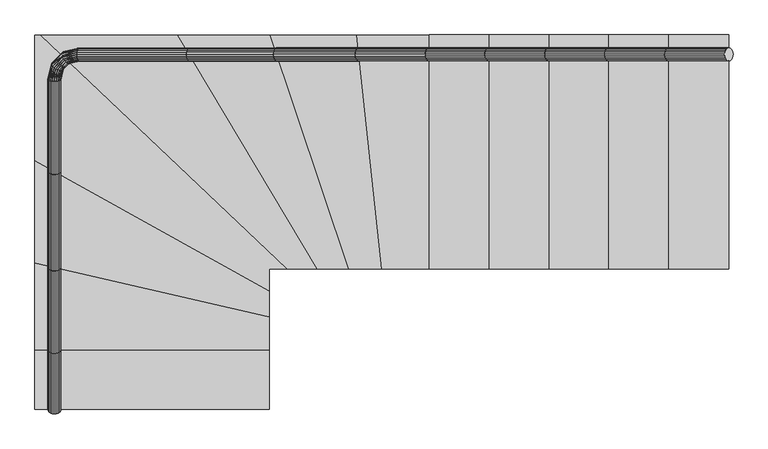
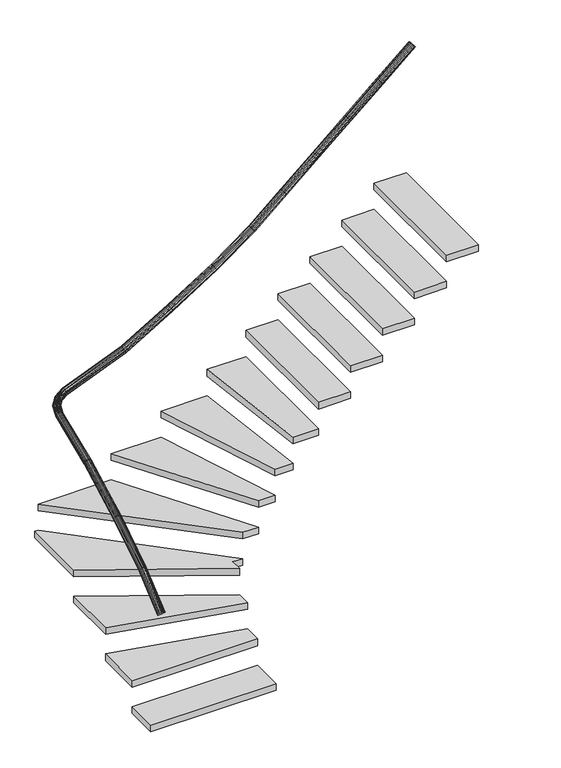
"""IFC4 building model written with IfcOpenShell, lengths in millimetres: stair geometry, 0_3d_modell."""

from ifc_helpers import new_model, si_unit, frame, origin, origin_with_axes, place, context, project, spatial, polyline, outline, extrude, faceted_brep, source, transform, mapped, element, save


def stair_df875d3e(model_context):
    return source(origin(), model_context, "Body", "SolidModel", [
        extrude(outline(polyline([(0.0, 246.9018591), (0.0, 579.8690495), (900.0, 373.9346688), (900.0, 246.9018591), (0.0, 246.9018591)])), frame((0.0, 0.0, 198.5714286), z_axis=(0.0, 0.0, 1.0), x_axis=(1.0, 0.0, 0.0)), (0.0, 0.0, 1.0), 50.0),
        extrude(outline(polyline([(0.0, 973.1970565), (0.0, 1456.9018591), (22.6704161, 1456.9018591), (970.0, 556.9018591), (900.0, 556.9018591), (900.0, 473.824936), (0.0, 973.1970565)])), frame((0.0, 0.0, 595.7142857), z_axis=(0.0, 0.0, 1.0), x_axis=(1.0, 0.0, 0.0)), (0.0, 0.0, 1.0), 50.0),
        extrude(outline(polyline([(548.8803485, 1456.9018591), (904.7220467, 1456.9018591), (1204.4816265, 556.9018591), (1084.3313864, 556.9018591), (548.8803485, 1456.9018591)])), frame((0.0, 0.0, 992.8571429), z_axis=(0.0, 0.0, 1.0), x_axis=(1.0, 0.0, 0.0)), (0.0, 0.0, 1.0), 50.0),
        faceted_brep([(98.7764129, 251.6675536, 1061.6862641), (100.0, 246.9018591, 1068.1306652), (98.7764129, 242.1361647, 1074.5750662), (95.2254249, 237.8369696, 1080.3886444), (89.6946313, 234.4251091, 1085.0023262), (82.7254249, 232.2345598, 1087.9644922), (75.0, 231.4797479, 1088.985185), (67.2745751, 232.2345598, 1087.9644922), (60.3053687, 234.4251091, 1085.0023262), (54.7745751, 237.8369696, 1080.3886444), (51.2235871, 242.1361647, 1074.5750662), (50.0, 246.9018591, 1068.1306652), (51.2235871, 251.6675536, 1061.6862641), (54.7745751, 255.9667486, 1055.872686), (60.3053687, 259.3786091, 1051.2590042), (67.2745751, 261.5691584, 1048.2968382), (75.0, 262.3239703, 1047.2761453), (82.7254249, 261.5691584, 1048.2968382), (89.6946313, 259.3786091, 1051.2590042), (95.2254249, 255.9667486, 1055.872686), (98.7764129, 558.6819455, 1273.6116568), (100.0, 562.7078511, 1266.7020937), (98.7764129, 566.7337566, 1259.7925307), (95.2254249, 570.3655785, 1253.5593239), (89.6946313, 573.2478087, 1248.6126229), (82.7254249, 575.0983143, 1245.4366454), (75.0, 575.7359551, 1244.3422781), (67.2745751, 575.0983143, 1245.4366454), (60.3053687, 573.2478087, 1248.6126229), (54.7745751, 570.3655785, 1253.5593239), (51.2235871, 566.7337566, 1259.7925307), (50.0, 562.7078511, 1266.7020937), (51.2235871, 558.6819455, 1273.6116568), (54.7745751, 555.0501237, 1279.8448636), (60.3053687, 552.1678935, 1284.7915646), (67.2745751, 550.3173878, 1287.9675421), (75.0, 549.679747, 1289.0619094), (82.7254249, 550.3173878, 1287.9675421), (89.6946313, 552.1678935, 1284.7915646), (95.2254249, 555.0501237, 1279.8448636)], [[[0, 1, 2, 3, 4, 5, 6, 7, 8, 9, 10, 11, 12, 13, 14, 15, 16, 17, 18, 19]], [[20, 21, 22, 23, 24, 25, 26, 27, 28, 29, 30, 31, 32, 33, 34, 35, 36, 37, 38, 39]], [[2, 1, 21, 20]], [[3, 2, 20, 39]], [[4, 3, 39, 38]], [[5, 4, 38, 37]], [[6, 5, 37, 36]], [[7, 6, 36, 35]], [[8, 7, 35, 34]], [[9, 8, 34, 33]], [[10, 9, 33, 32]], [[11, 10, 32, 31]], [[12, 11, 31, 30]], [[13, 12, 30, 29]], [[14, 13, 29, 28]], [[15, 14, 28, 27]], [[16, 15, 27, 26]], [[17, 16, 26, 25]], [[18, 17, 25, 24]], [[19, 18, 24, 23]], [[0, 19, 23, 22]], [[1, 0, 22, 21]]]),
        extrude(outline(polyline([(1974.6018366, 1456.9018591), (2204.6018366, 1456.9018591), (2204.6018366, 556.9018591), (1974.6018366, 556.9018591), (1974.6018366, 1456.9018591)])), frame((0.0, 0.0, 1985.7142857), z_axis=(0.0, 0.0, 1.0), x_axis=(1.0, 0.0, 0.0)), (0.0, 0.0, 1.0), 50.0),
        extrude(outline(polyline([(1.2235871, -7.9923214), (0.0, 0.0), (1.2235871, 7.9923214), (4.7745752, 15.2022986), (10.3053687, 20.9241691), (17.2745752, 24.5978359), (25.0, 25.8636953), (32.7254249, 24.5978359), (39.6946313, 20.9241691), (45.2254249, 15.2022986), (48.7764129, 7.9923214), (50.0, 0.0), (48.7764129, -7.9923214), (45.2254249, -15.2022986), (39.6946313, -20.9241691), (32.7254249, -24.5978359), (25.0, -25.8636953), (17.2745752, -24.5978359), (10.3053687, -20.9241691), (4.7745752, -15.2022986), (1.2235871, -7.9923214)])), frame((2204.6018366, 1356.9018591, 3053.8449509), z_axis=(0.7569287102857765, 0.0, 0.6534974579484691), x_axis=(0.0, 1.0, 0.0)), (0.0, 0.0, 1.0), 303.8595272),
        faceted_brep([(98.7764129, 566.7337566, 1259.7925307), (100.0, 562.7078511, 1266.7020937), (98.7764129, 558.6819455, 1273.6116568), (95.2254249, 555.0501237, 1279.8448636), (89.6946313, 552.1678935, 1284.7915646), (82.7254249, 550.3173878, 1287.9675421), (75.0, 549.679747, 1289.0619094), (67.2745751, 550.3173878, 1287.9675421), (60.3053687, 552.1678935, 1284.7915646), (54.7745751, 555.0501237, 1279.8448636), (51.2235871, 558.6819455, 1273.6116568), (50.0, 562.7078511, 1266.7020937), (51.2235871, 566.7337566, 1259.7925307), (54.7745751, 570.3655785, 1253.5593239), (60.3053687, 573.2478087, 1248.6126229), (67.2745751, 575.0983143, 1245.4366454), (75.0, 575.7359551, 1244.3422781), (82.7254249, 575.0983143, 1245.4366454), (89.6946313, 573.2478087, 1248.6126229), (95.2254249, 570.3655785, 1253.5593239), (98.7764129, 928.1440687, 1472.4992177), (100.0, 931.5827131, 1465.2735223), (98.7764129, 935.0213576, 1458.0478269), (95.2254249, 938.1234035, 1451.529433), (89.6946313, 940.5852011, 1446.3564062), (82.7254249, 942.1657724, 1443.0351186), (75.0, 942.7104002, 1441.8906809), (67.2745751, 942.1657724, 1443.0351186), (60.3053687, 940.5852011, 1446.3564062), (54.7745751, 938.1234035, 1451.529433), (51.2235871, 935.0213576, 1458.0478269), (50.0, 931.5827131, 1465.2735223), (51.2235871, 928.1440687, 1472.4992177), (54.7745751, 925.0420228, 1479.0176117), (60.3053687, 922.5802252, 1484.1906384), (67.2745751, 920.9996538, 1487.511926), (75.0, 920.4550261, 1488.6563638), (82.7254249, 920.9996538, 1487.511926), (89.6946313, 922.5802252, 1484.1906384), (95.2254249, 925.0420228, 1479.0176117)], [[[0, 1, 2, 3, 4, 5, 6, 7, 8, 9, 10, 11, 12, 13, 14, 15, 16, 17, 18, 19]], [[20, 21, 22, 23, 24, 25, 26, 27, 28, 29, 30, 31, 32, 33, 34, 35, 36, 37, 38, 39]], [[2, 1, 21, 20]], [[3, 2, 20, 39]], [[4, 3, 39, 38]], [[5, 4, 38, 37]], [[6, 5, 37, 36]], [[7, 6, 36, 35]], [[8, 7, 35, 34]], [[9, 8, 34, 33]], [[10, 9, 33, 32]], [[11, 10, 32, 31]], [[12, 11, 31, 30]], [[13, 12, 30, 29]], [[14, 13, 29, 28]], [[15, 14, 28, 27]], [[16, 15, 27, 26]], [[17, 16, 26, 25]], [[18, 17, 25, 24]], [[19, 18, 24, 23]], [[0, 19, 23, 22]], [[1, 0, 22, 21]]]),
        extrude(outline(polyline([(2434.6018366, 1456.9018591), (2664.6018366, 1456.9018591), (2664.6018366, 556.9018591), (2434.6018366, 556.9018591), (2434.6018366, 1456.9018591)])), frame((0.0, 0.0, 2382.8571429), z_axis=(0.0, 0.0, 1.0), x_axis=(1.0, 0.0, 0.0)), (0.0, 0.0, 1.0), 50.0),
        faceted_brep([(98.7764129, 935.0213576, 1458.0478269), (100.0, 931.5827131, 1465.2735223), (98.7764129, 928.1440687, 1472.4992177), (95.2254249, 925.0420228, 1479.0176117), (89.6946313, 922.5802252, 1484.1906384), (82.7254249, 920.9996538, 1487.511926), (75.0, 920.4550261, 1488.6563638), (67.2745751, 920.9996538, 1487.511926), (60.3053687, 922.5802252, 1484.1906384), (54.7745751, 925.0420228, 1479.0176117), (51.2235871, 928.1440687, 1472.4992177), (50.0, 931.5827131, 1465.2735223), (51.2235871, 935.0213576, 1458.0478269), (54.7745751, 938.1234035, 1451.529433), (60.3053687, 940.5852011, 1446.3564062), (67.2745751, 942.1657724, 1443.0351186), (75.0, 942.7104002, 1441.8906809), (82.7254249, 942.1657724, 1443.0351186), (89.6946313, 940.5852011, 1446.3564062), (95.2254249, 938.1234035, 1451.529433), (98.7764129, 1283.3224302, 1620.3777918), (100.0, 1286.3944101, 1612.9994356), (98.7764129, 1289.46639, 1605.6210794), (95.2254249, 1292.2376632, 1598.9649681), (89.6946313, 1294.436958, 1593.6826483), (82.7254249, 1295.8489921, 1590.2911902), (75.0, 1296.335546, 1589.1225734), (67.2745751, 1295.8489921, 1590.2911902), (60.3053687, 1294.436958, 1593.6826483), (54.7745751, 1292.2376632, 1598.9649681), (51.2235871, 1289.46639, 1605.6210794), (50.0, 1286.3944101, 1612.9994356), (51.2235871, 1283.3224302, 1620.3777918), (54.7745751, 1280.5511571, 1627.0339031), (60.3053687, 1278.3518623, 1632.3162229), (67.2745751, 1276.9398281, 1635.707681), (75.0, 1276.4532743, 1636.8762979), (82.7254249, 1276.9398281, 1635.707681), (89.6946313, 1278.3518623, 1632.3162229), (95.2254249, 1280.5511571, 1627.0339031)], [[[0, 1, 2, 3, 4, 5, 6, 7, 8, 9, 10, 11, 12, 13, 14, 15, 16, 17, 18, 19]], [[20, 21, 22, 23, 24, 25, 26, 27, 28, 29, 30, 31, 32, 33, 34, 35, 36, 37, 38, 39]], [[2, 1, 21, 20]], [[3, 2, 20, 39]], [[4, 3, 39, 38]], [[5, 4, 38, 37]], [[6, 5, 37, 36]], [[7, 6, 36, 35]], [[8, 7, 35, 34]], [[9, 8, 34, 33]], [[10, 9, 33, 32]], [[11, 10, 32, 31]], [[12, 11, 31, 30]], [[13, 12, 30, 29]], [[14, 13, 29, 28]], [[15, 14, 28, 27]], [[16, 15, 27, 26]], [[17, 16, 26, 25]], [[18, 17, 25, 24]], [[19, 18, 24, 23]], [[0, 19, 23, 22]], [[1, 0, 22, 21]]]),
        faceted_brep([(1249.3489942, 1358.1254462, 2252.9513864), (1244.8437697, 1356.9018591, 2259.5592366), (1240.3385453, 1358.1254462, 2266.1670868), (1236.2743236, 1361.6764343, 2272.1281145), (1233.048939, 1367.2072278, 2276.858813), (1230.9781146, 1374.1764343, 2279.8961083), (1230.2645572, 1381.9018591, 2280.942689), (1230.9781146, 1389.627284, 2279.8961083), (1233.048939, 1396.5964904, 2276.858813), (1236.2743236, 1402.127284, 2272.1281145), (1240.3385453, 1405.678272, 2266.1670868), (1244.8437697, 1406.9018591, 2259.5592366), (1249.3489942, 1405.678272, 2252.9513864), (1253.4132159, 1402.127284, 2246.9903587), (1256.6386004, 1396.5964904, 2242.2596602), (1258.7094248, 1389.627284, 2239.2223649), (1259.4229823, 1381.9018591, 2238.1757842), (1258.7094248, 1374.1764343, 2239.2223649), (1256.6386004, 1367.2072278, 2242.2596602), (1253.4132159, 1361.6764343, 2246.9903587), (1509.6138519, 1358.1254462, 2464.383151), (1514.6018366, 1356.9018591, 2458.1306652), (1519.5898213, 1358.1254462, 2451.8781793), (1524.0895473, 1361.6764343, 2446.2377304), (1527.6605501, 1367.2072278, 2441.7614447), (1529.9532751, 1374.1764343, 2438.8874925), (1530.7432942, 1381.9018591, 2437.897196), (1529.9532751, 1389.627284, 2438.8874925), (1527.6605501, 1396.5964904, 2441.7614447), (1524.0895473, 1402.127284, 2446.2377304), (1519.5898213, 1405.678272, 2451.8781793), (1514.6018366, 1406.9018591, 2458.1306652), (1509.6138519, 1405.678272, 2464.383151), (1505.1141259, 1402.127284, 2470.0236), (1501.5431231, 1396.5964904, 2474.4998856), (1499.2503981, 1389.627284, 2477.3738379), (1498.460379, 1381.9018591, 2478.3641344), (1499.2503981, 1374.1764343, 2477.3738379), (1501.5431231, 1367.2072278, 2474.4998856), (1505.1141259, 1361.6764343, 2470.0236)], [[[0, 1, 2, 3, 4, 5, 6, 7, 8, 9, 10, 11, 12, 13, 14, 15, 16, 17, 18, 19]], [[20, 21, 22, 23, 24, 25, 26, 27, 28, 29, 30, 31, 32, 33, 34, 35, 36, 37, 38, 39]], [[2, 1, 21, 20]], [[3, 2, 20, 39]], [[4, 3, 39, 38]], [[5, 4, 38, 37]], [[6, 5, 37, 36]], [[7, 6, 36, 35]], [[8, 7, 35, 34]], [[9, 8, 34, 33]], [[10, 9, 33, 32]], [[11, 10, 32, 31]], [[12, 11, 31, 30]], [[13, 12, 30, 29]], [[14, 13, 29, 28]], [[15, 14, 28, 27]], [[16, 15, 27, 26]], [[17, 16, 26, 25]], [[18, 17, 25, 24]], [[19, 18, 24, 23]], [[0, 19, 23, 22]], [[1, 0, 22, 21]]]),
        extrude(outline(polyline([(1.2235871, -7.9923214), (0.0, 0.0), (1.2235871, 7.9923214), (4.7745752, 15.2022986), (10.3053687, 20.924169), (17.2745752, 24.5978359), (25.0, 25.8636953), (32.7254249, 24.5978359), (39.6946313, 20.924169), (45.2254249, 15.2022986), (48.7764129, 7.9923214), (50.0, 0.0), (48.7764129, -7.9923214), (45.2254249, -15.2022986), (39.6946313, -20.9241691), (32.7254249, -24.597836), (25.0, -25.8636953), (17.2745752, -24.597836), (10.3053687, -20.9241691), (4.7745752, -15.2022986), (1.2235871, -7.9923214)])), frame((2434.6018366, 1356.9018591, 3252.4163795), z_axis=(0.7569287102857786, 0.0, 0.6534974579484667), x_axis=(0.0, 1.0, 0.0)), (0.0, 0.0, 1.0), 303.8595272),
        extrude(outline(polyline([(0.0, 579.8690495), (0.0, 973.1970565), (900.0, 473.824936), (900.0, 373.9346688), (0.0, 579.8690495)])), frame((0.0, 0.0, 397.1428571), z_axis=(0.0, 0.0, 1.0), x_axis=(1.0, 0.0, 0.0)), (0.0, 0.0, 1.0), 50.0),
        extrude(outline(polyline([(22.6704161, 1456.9018591), (548.8803485, 1456.9018591), (1084.3313864, 556.9018591), (970.0, 556.9018591), (22.6704161, 1456.9018591)])), frame((0.0, 0.0, 794.2857143), z_axis=(0.0, 0.0, 1.0), x_axis=(1.0, 0.0, 0.0)), (0.0, 0.0, 1.0), 50.0),
        extrude(outline(polyline([(1.2235871, -7.9923214), (0.0, 0.0), (1.2235871, 7.9923214), (4.7745752, 15.2022987), (10.3053687, 20.9241691), (17.2745752, 24.597836), (25.0, 25.8636953), (32.7254249, 24.597836), (39.6946313, 20.9241691), (45.2254249, 15.2022987), (48.7764129, 7.9923214), (50.0, 0.0), (48.7764129, -7.9923214), (45.2254249, -15.2022986), (39.6946313, -20.924169), (32.7254249, -24.5978359), (25.0, -25.8636953), (17.2745752, -24.5978359), (10.3053687, -20.924169), (4.7745752, -15.2022986), (1.2235871, -7.9923214)])), frame((1744.6018366, 1356.9018591, 2656.7020937), z_axis=(0.7569287102857375, 0.0, 0.6534974579485143), x_axis=(0.0, 1.0, 0.0)), (0.0, 0.0, 1.0), 303.8595272),
        faceted_brep([(933.8654844, 1358.1254462, 2054.1646194), (929.7020117, 1356.9018591, 2060.987808), (925.538539, 1358.1254462, 2067.8109967), (921.782616, 1361.6764343, 2073.966284), (918.8018987, 1367.2072278, 2078.8511477), (916.8881603, 1374.1764343, 2081.9874233), (916.228731, 1381.9018591, 2083.0681102), (916.8881603, 1389.627284, 2081.9874233), (918.8018987, 1396.5964904, 2078.8511477), (921.782616, 1402.127284, 2073.966284), (925.538539, 1405.678272, 2067.8109967), (929.7020117, 1406.9018591, 2060.987808), (933.8654844, 1405.678272, 2054.1646194), (937.6214074, 1402.127284, 2048.009332), (940.6021247, 1396.5964904, 2043.1244683), (942.515863, 1389.627284, 2039.9881928), (943.1752923, 1381.9018591, 2038.9075058), (942.515863, 1374.1764343, 2039.9881928), (940.6021247, 1367.2072278, 2043.1244683), (937.6214074, 1361.6764343, 2048.009332), (1240.3385453, 1358.1254462, 2266.1670868), (1244.8437697, 1356.9018591, 2259.5592366), (1249.3489942, 1358.1254462, 2252.9513864), (1253.4132159, 1361.6764343, 2246.9903587), (1256.6386004, 1367.2072278, 2242.2596602), (1258.7094248, 1374.1764343, 2239.2223649), (1259.4229823, 1381.9018591, 2238.1757842), (1258.7094248, 1389.627284, 2239.2223649), (1256.6386004, 1396.5964904, 2242.2596602), (1253.4132159, 1402.127284, 2246.9903587), (1249.3489942, 1405.678272, 2252.9513864), (1244.8437697, 1406.9018591, 2259.5592366), (1240.3385453, 1405.678272, 2266.1670868), (1236.2743236, 1402.127284, 2272.1281145), (1233.048939, 1396.5964904, 2276.858813), (1230.9781146, 1389.627284, 2279.8961083), (1230.2645572, 1381.9018591, 2280.942689), (1230.9781146, 1374.1764343, 2279.8961083), (1233.048939, 1367.2072278, 2276.858813), (1236.2743236, 1361.6764343, 2272.1281145)], [[[0, 1, 2, 3, 4, 5, 6, 7, 8, 9, 10, 11, 12, 13, 14, 15, 16, 17, 18, 19]], [[20, 21, 22, 23, 24, 25, 26, 27, 28, 29, 30, 31, 32, 33, 34, 35, 36, 37, 38, 39]], [[2, 1, 21, 20]], [[3, 2, 20, 39]], [[4, 3, 39, 38]], [[5, 4, 38, 37]], [[6, 5, 37, 36]], [[7, 6, 36, 35]], [[8, 7, 35, 34]], [[9, 8, 34, 33]], [[10, 9, 33, 32]], [[11, 10, 32, 31]], [[12, 11, 31, 30]], [[13, 12, 30, 29]], [[14, 13, 29, 28]], [[15, 14, 28, 27]], [[16, 15, 27, 26]], [[17, 16, 26, 25]], [[18, 17, 25, 24]], [[19, 18, 24, 23]], [[0, 19, 23, 22]], [[1, 0, 22, 21]]]),
        faceted_brep([(597.0493296, 1358.1254462, 1855.2297082), (593.5012683, 1356.9018591, 1862.4163795), (589.9532071, 1358.1254462, 1869.6030507), (586.7524548, 1361.6764343, 1876.0862405), (584.2123234, 1367.2072278, 1881.231329), (582.5814586, 1374.1764343, 1884.5346792), (582.019501, 1381.9018591, 1885.6729361), (582.5814586, 1389.627284, 1884.5346792), (584.2123234, 1396.5964904, 1881.231329), (586.7524548, 1402.127284, 1876.0862405), (589.9532071, 1405.678272, 1869.6030507), (593.5012683, 1406.9018591, 1862.4163795), (597.0493296, 1405.678272, 1855.2297082), (600.2500819, 1402.127284, 1848.7465184), (602.7902133, 1396.5964904, 1843.6014299), (604.421078, 1389.627284, 1840.2980797), (604.9830357, 1381.9018591, 1839.1598228), (604.421078, 1374.1764343, 1840.2980797), (602.7902133, 1367.2072278, 1843.6014299), (600.2500819, 1361.6764343, 1848.7465184), (925.538539, 1358.1254462, 2067.8109967), (929.7020117, 1356.9018591, 2060.987808), (933.8654844, 1358.1254462, 2054.1646194), (937.6214074, 1361.6764343, 2048.009332), (940.6021247, 1367.2072278, 2043.1244683), (942.515863, 1374.1764343, 2039.9881928), (943.1752923, 1381.9018591, 2038.9075058), (942.515863, 1389.627284, 2039.9881928), (940.6021247, 1396.5964904, 2043.1244683), (937.6214074, 1402.127284, 2048.009332), (933.8654844, 1405.678272, 2054.1646194), (929.7020117, 1406.9018591, 2060.987808), (925.538539, 1405.678272, 2067.8109967), (921.782616, 1402.127284, 2073.966284), (918.8018987, 1396.5964904, 2078.8511477), (916.8881603, 1389.627284, 2081.9874233), (916.228731, 1381.9018591, 2083.0681102), (916.8881603, 1374.1764343, 2081.9874233), (918.8018987, 1367.2072278, 2078.8511477), (921.782616, 1361.6764343, 2073.966284)], [[[0, 1, 2, 3, 4, 5, 6, 7, 8, 9, 10, 11, 12, 13, 14, 15, 16, 17, 18, 19]], [[20, 21, 22, 23, 24, 25, 26, 27, 28, 29, 30, 31, 32, 33, 34, 35, 36, 37, 38, 39]], [[2, 1, 21, 20]], [[3, 2, 20, 39]], [[4, 3, 39, 38]], [[5, 4, 38, 37]], [[6, 5, 37, 36]], [[7, 6, 36, 35]], [[8, 7, 35, 34]], [[9, 8, 34, 33]], [[10, 9, 33, 32]], [[11, 10, 32, 31]], [[12, 11, 31, 30]], [[13, 12, 30, 29]], [[14, 13, 29, 28]], [[15, 14, 28, 27]], [[16, 15, 27, 26]], [[17, 16, 26, 25]], [[18, 17, 25, 24]], [[19, 18, 24, 23]], [[0, 19, 23, 22]], [[1, 0, 22, 21]]]),
        faceted_brep([(98.7764129, 1289.46639, 1605.6210794), (100.0, 1286.3944101, 1612.9994356), (98.7764129, 1283.3224302, 1620.3777918), (95.2254249, 1280.5511571, 1627.0339031), (89.6946313, 1278.3518623, 1632.3162229), (82.7254249, 1276.9398281, 1635.707681), (75.0, 1276.4532743, 1636.8762979), (67.2745751, 1276.9398281, 1635.707681), (60.3053687, 1278.3518623, 1632.3162229), (54.7745751, 1280.5511571, 1627.0339031), (51.2235871, 1283.3224302, 1620.3777918), (50.0, 1286.3944101, 1612.9994356), (51.2235871, 1289.46639, 1605.6210794), (54.7745751, 1292.2376632, 1598.9649681), (60.3053687, 1294.436958, 1593.6826483), (67.2745751, 1295.8489921, 1590.2911902), (75.0, 1296.335546, 1589.1225734), (82.7254249, 1295.8489921, 1590.2911902), (89.6946313, 1294.436958, 1593.6826483), (95.2254249, 1292.2376632, 1598.9649681), (108.8679012, 1324.8479302, 1638.9123688), (105.9144976, 1321.9997167, 1645.879395), (101.1034244, 1320.6050585, 1652.1644401), (94.9056231, 1320.8004745, 1657.1522801), (87.9277774, 1322.5668359, 1660.3546705), (80.8529277, 1325.7312391, 1661.4581391), (74.3736094, 1329.9839302, 1660.3546705), (69.1240635, 1334.9086261, 1657.1522801), (65.6181519, 1340.0232633, 1652.1644401), (64.1990579, 1344.8271855, 1645.879395), (65.0056921, 1348.8501513, 1638.9123688), (67.9590957, 1351.6983647, 1631.9453426), (72.7701688, 1353.0930229, 1625.6602975), (78.9679702, 1352.8976069, 1620.6724574), (85.9458159, 1351.1312455, 1617.470067), (93.0206656, 1347.9668423, 1616.3665985), (99.4999839, 1343.7141513, 1617.470067), (104.7495298, 1338.7894554, 1620.6724574), (108.2554414, 1333.6748181, 1625.6602975), (109.6745354, 1328.870896, 1631.9453426), (132.1170605, 1348.0291684, 1666.2859781), (128.1175831, 1347.2454175, 1673.2691208), (123.3397137, 1348.6878091, 1679.5687049), (118.2511434, 1352.215152, 1684.5680831), (113.3499769, 1357.4821652, 1687.7778814), (109.1159746, 1363.9732768, 1688.8839026), (105.96359, 1371.0530916, 1687.7778814), (104.2014005, 1378.028588, 1684.5680831), (104.0019016, 1384.2169558, 1679.5687049), (105.3846216, 1389.0124344, 1673.2691208), (108.2142101, 1391.9456089, 1666.2859781), (112.2136875, 1392.7293599, 1659.3028354), (116.9915569, 1391.2869683, 1653.0032514), (122.0801271, 1387.7596254, 1648.0038732), (126.9812936, 1382.4926122, 1644.7940748), (131.215296, 1376.0015006, 1643.6880537), (134.3676806, 1368.9216857, 1644.7940748), (136.1298701, 1361.9461894, 1648.0038732), (136.329369, 1355.7578216, 1653.0032514), (134.946649, 1350.962343, 1659.3028354), (170.8141891, 1356.9018591, 1691.7803901), (167.8223333, 1358.1254462, 1699.1915978), (165.1233413, 1361.6764343, 1705.8773449), (162.981409, 1367.2072278, 1711.1831838), (161.6062039, 1374.1764343, 1714.5897421), (161.1323405, 1381.9018591, 1715.7635621), (161.6062039, 1389.627284, 1714.5897421), (162.981409, 1396.5964904, 1711.1831838), (165.1233413, 1402.127284, 1705.8773449), (167.8223333, 1405.678272, 1699.1915978), (170.8141891, 1406.9018591, 1691.7803901), (173.8060448, 1405.678272, 1684.3691823), (176.5050369, 1402.127284, 1677.6834352), (178.6469691, 1396.5964904, 1672.3775963), (180.0221742, 1389.627284, 1668.971038), (180.4960376, 1381.9018591, 1667.797218), (180.0221742, 1374.1764343, 1668.971038), (178.6469691, 1367.2072278, 1672.3775963), (176.5050369, 1361.6764343, 1677.6834352), (173.8060448, 1358.1254462, 1684.3691823), (589.9532071, 1358.1254462, 1869.6030507), (593.5012683, 1356.9018591, 1862.4163795), (597.0493296, 1358.1254462, 1855.2297082), (600.2500819, 1361.6764343, 1848.7465184), (602.7902133, 1367.2072278, 1843.6014299), (604.421078, 1374.1764343, 1840.2980797), (604.9830357, 1381.9018591, 1839.1598228), (604.421078, 1389.627284, 1840.2980797), (602.7902133, 1396.5964904, 1843.6014299), (600.2500819, 1402.127284, 1848.7465184), (597.0493296, 1405.678272, 1855.2297082), (593.5012683, 1406.9018591, 1862.4163795), (589.9532071, 1405.678272, 1869.6030507), (586.7524548, 1402.127284, 1876.0862405), (584.2123234, 1396.5964904, 1881.231329), (582.5814586, 1389.627284, 1884.5346792), (582.019501, 1381.9018591, 1885.6729361), (582.5814586, 1374.1764343, 1884.5346792), (584.2123234, 1367.2072278, 1881.231329), (586.7524548, 1361.6764343, 1876.0862405)], [[[0, 1, 2, 3, 4, 5, 6, 7, 8, 9, 10, 11, 12, 13, 14, 15, 16, 17, 18, 19]], [[2, 1, 20]], [[21, 2, 20]], [[3, 2, 21]], [[22, 3, 21]], [[4, 3, 22]], [[23, 4, 22]], [[5, 4, 23]], [[24, 5, 23]], [[6, 5, 24]], [[25, 6, 24]], [[7, 6, 25]], [[26, 7, 25]], [[8, 7, 26]], [[27, 8, 26]], [[9, 8, 27]], [[28, 9, 27]], [[10, 9, 28]], [[29, 10, 28]], [[11, 10, 29]], [[30, 11, 29]], [[12, 11, 30]], [[31, 12, 30]], [[13, 12, 31]], [[32, 13, 31]], [[14, 13, 32]], [[33, 14, 32]], [[15, 14, 33]], [[34, 15, 33]], [[16, 15, 34]], [[35, 16, 34]], [[17, 16, 35]], [[36, 17, 35]], [[18, 17, 36]], [[37, 18, 36]], [[19, 18, 37]], [[38, 19, 37]], [[0, 19, 38]], [[39, 0, 38]], [[1, 0, 39]], [[20, 1, 39]], [[21, 20, 40]], [[41, 21, 40]], [[22, 21, 41]], [[42, 22, 41]], [[23, 22, 42]], [[43, 23, 42]], [[24, 23, 43]], [[44, 24, 43]], [[25, 24, 44]], [[45, 25, 44]], [[26, 25, 45]], [[46, 26, 45]], [[27, 26, 46]], [[47, 27, 46]], [[28, 27, 47]], [[48, 28, 47]], [[29, 28, 48]], [[49, 29, 48]], [[30, 29, 49]], [[50, 30, 49]], [[31, 30, 50]], [[51, 31, 50]], [[32, 31, 51]], [[52, 32, 51]], [[33, 32, 52]], [[53, 33, 52]], [[34, 33, 53]], [[54, 34, 53]], [[35, 34, 54]], [[55, 35, 54]], [[36, 35, 55]], [[56, 36, 55]], [[37, 36, 56]], [[57, 37, 56]], [[38, 37, 57]], [[58, 38, 57]], [[39, 38, 58]], [[59, 39, 58]], [[20, 39, 59]], [[40, 20, 59]], [[41, 40, 60]], [[61, 41, 60]], [[42, 41, 61]], [[62, 42, 61]], [[43, 42, 62]], [[63, 43, 62]], [[44, 43, 63]], [[64, 44, 63]], [[45, 44, 64]], [[65, 45, 64]], [[46, 45, 65]], [[66, 46, 65]], [[47, 46, 66]], [[67, 47, 66]], [[48, 47, 67]], [[68, 48, 67]], [[49, 48, 68]], [[69, 49, 68]], [[50, 49, 69]], [[70, 50, 69]], [[51, 50, 70]], [[71, 51, 70]], [[52, 51, 71]], [[72, 52, 71]], [[53, 52, 72]], [[73, 53, 72]], [[54, 53, 73]], [[74, 54, 73]], [[55, 54, 74]], [[75, 55, 74]], [[56, 55, 75]], [[76, 56, 75]], [[57, 56, 76]], [[77, 57, 76]], [[58, 57, 77]], [[78, 58, 77]], [[59, 58, 78]], [[79, 59, 78]], [[40, 59, 79]], [[60, 40, 79]], [[80, 81, 82, 83, 84, 85, 86, 87, 88, 89, 90, 91, 92, 93, 94, 95, 96, 97, 98, 99]], [[61, 60, 81, 80]], [[62, 61, 80, 99]], [[63, 62, 99, 98]], [[64, 63, 98, 97]], [[65, 64, 97, 96]], [[66, 65, 96, 95]], [[67, 66, 95, 94]], [[68, 67, 94, 93]], [[69, 68, 93, 92]], [[70, 69, 92, 91]], [[71, 70, 91, 90]], [[72, 71, 90, 89]], [[73, 72, 89, 88]], [[74, 73, 88, 87]], [[75, 74, 87, 86]], [[76, 75, 86, 85]], [[77, 76, 85, 84]], [[78, 77, 84, 83]], [[79, 78, 83, 82]], [[60, 79, 82, 81]]]),
        extrude(outline(polyline([(1.2235871, -7.9923214), (0.0, 0.0), (1.2235871, 7.9923214), (4.7745752, 15.2022986), (10.3053687, 20.9241691), (17.2745752, 24.5978359), (25.0, 25.8636953), (32.7254249, 24.5978359), (39.6946313, 20.9241691), (45.2254249, 15.2022986), (48.7764129, 7.9923214), (50.0, 0.0), (48.7764129, -7.9923214), (45.2254249, -15.2022986), (39.6946313, -20.924169), (32.7254249, -24.5978359), (25.0, -25.8636953), (17.2745752, -24.5978359), (10.3053687, -20.924169), (4.7745752, -15.2022986), (1.2235871, -7.9923214)])), frame((1974.6018366, 1356.9018591, 2855.2735223), z_axis=(0.7569287102857345, 0.0, 0.6534974579485179), x_axis=(0.0, 1.0, 0.0)), (0.0, 0.0, 1.0), 303.8595272),
        extrude(outline(polyline([(0.0, 16.9018591), (0.0, 246.9018591), (900.0, 246.9018591), (900.0, 16.9018591), (0.0, 16.9018591)])), origin_with_axes(), (0.0, 0.0, 1.0), 50.0),
        extrude(outline(polyline([(1744.6018366, 1456.9018591), (1974.6018366, 1456.9018591), (1974.6018366, 556.9018591), (1744.6018366, 556.9018591), (1744.6018366, 1456.9018591)])), frame((0.0, 0.0, 1787.1428571), z_axis=(0.0, 0.0, 1.0), x_axis=(1.0, 0.0, 0.0)), (0.0, 0.0, 1.0), 50.0),
        faceted_brep([(98.7764129, 22.1248208, 863.5096191), (100.0, 16.9018591, 869.5592366), (98.7764129, 11.6788974, 875.6088541), (95.2254249, 6.9671956, 881.0662929), (89.6946313, 3.2279679, 885.3973409), (82.7254249, 0.8272359, 888.1780448), (75.0, 0.0, 889.1362101), (67.2745751, 0.8272359, 888.1780448), (60.3053687, 3.2279679, 885.3973409), (54.7745751, 6.9671956, 881.0662929), (51.2235871, 11.6788974, 875.6088541), (50.0, 16.9018591, 869.5592366), (51.2235871, 22.1248208, 863.5096191), (54.7745751, 26.8365226, 858.0521803), (60.3053687, 30.5757504, 853.7211323), (67.2745751, 32.9764824, 850.9404284), (75.0, 33.8037182, 849.9822631), (82.7254249, 32.9764824, 850.9404284), (89.6946313, 30.5757504, 853.7211323), (95.2254249, 26.8365226, 858.0521803), (98.7764129, 242.1361647, 1074.5750662), (100.0, 246.9018591, 1068.1306652), (98.7764129, 251.6675536, 1061.6862641), (95.2254249, 255.9667486, 1055.872686), (89.6946313, 259.3786091, 1051.2590042), (82.7254249, 261.5691584, 1048.2968382), (75.0, 262.3239703, 1047.2761453), (67.2745751, 261.5691584, 1048.2968382), (60.3053687, 259.3786091, 1051.2590042), (54.7745751, 255.9667486, 1055.872686), (51.2235871, 251.6675536, 1061.6862641), (50.0, 246.9018591, 1068.1306652), (51.2235871, 242.1361647, 1074.5750662), (54.7745751, 237.8369696, 1080.3886444), (60.3053687, 234.4251091, 1085.0023262), (67.2745751, 232.2345598, 1087.9644922), (75.0, 231.4797479, 1088.985185), (82.7254249, 232.2345598, 1087.9644922), (89.6946313, 234.4251091, 1085.0023262), (95.2254249, 237.8369696, 1080.3886444)], [[[0, 1, 2, 3, 4, 5, 6, 7, 8, 9, 10, 11, 12, 13, 14, 15, 16, 17, 18, 19]], [[20, 21, 22, 23, 24, 25, 26, 27, 28, 29, 30, 31, 32, 33, 34, 35, 36, 37, 38, 39]], [[2, 1, 21, 20]], [[3, 2, 20, 39]], [[4, 3, 39, 38]], [[5, 4, 38, 37]], [[6, 5, 37, 36]], [[7, 6, 36, 35]], [[8, 7, 35, 34]], [[9, 8, 34, 33]], [[10, 9, 33, 32]], [[11, 10, 32, 31]], [[12, 11, 31, 30]], [[13, 12, 30, 29]], [[14, 13, 29, 28]], [[15, 14, 28, 27]], [[16, 15, 27, 26]], [[17, 16, 26, 25]], [[18, 17, 25, 24]], [[19, 18, 24, 23]], [[0, 19, 23, 22]], [[1, 0, 22, 21]]]),
        extrude(outline(polyline([(2204.6018366, 1456.9018591), (2434.6018366, 1456.9018591), (2434.6018366, 556.9018591), (2204.6018366, 556.9018591), (2204.6018366, 1456.9018591)])), frame((0.0, 0.0, 2184.2857143), z_axis=(0.0, 0.0, 1.0), x_axis=(1.0, 0.0, 0.0)), (0.0, 0.0, 1.0), 50.0),
        extrude(outline(polyline([(1514.6018366, 1456.9018591), (1744.6018366, 1456.9018591), (1744.6018366, 556.9018591), (1514.6018366, 556.9018591), (1514.6018366, 1456.9018591)])), frame((0.0, 0.0, 1588.5714286), z_axis=(0.0, 0.0, 1.0), x_axis=(1.0, 0.0, 0.0)), (0.0, 0.0, 1.0), 50.0),
        extrude(outline(polyline([(1236.8921564, 1456.9018591), (1514.6018366, 1456.9018591), (1514.6018366, 556.9018591), (1332.3115168, 556.9018591), (1236.8921564, 1456.9018591)])), frame((0.0, 0.0, 1390.0), z_axis=(0.0, 0.0, 1.0), x_axis=(1.0, 0.0, 0.0)), (0.0, 0.0, 1.0), 50.0),
        extrude(outline(polyline([(904.7220467, 1456.9018591), (1236.8921564, 1456.9018591), (1332.3115168, 556.9018591), (1204.4816265, 556.9018591), (904.7220467, 1456.9018591)])), frame((0.0, 0.0, 1191.4285714), z_axis=(0.0, 0.0, 1.0), x_axis=(1.0, 0.0, 0.0)), (0.0, 0.0, 1.0), 50.0),
        faceted_brep([(1519.5898213, 1358.1254462, 2451.8781793), (1514.6018366, 1356.9018591, 2458.1306652), (1509.6138519, 1358.1254462, 2464.383151), (1505.1141259, 1361.6764343, 2470.0236), (1501.5431231, 1367.2072278, 2474.4998856), (1499.2503981, 1374.1764343, 2477.3738379), (1498.460379, 1381.9018591, 2478.3641344), (1499.2503981, 1389.627284, 2477.3738379), (1501.5431231, 1396.5964904, 2474.4998856), (1505.1141259, 1402.127284, 2470.0236), (1509.6138519, 1405.678272, 2464.383151), (1514.6018366, 1406.9018591, 2458.1306652), (1519.5898213, 1405.678272, 2451.8781793), (1524.0895473, 1402.127284, 2446.2377304), (1527.6605501, 1396.5964904, 2441.7614447), (1529.9532751, 1389.627284, 2438.8874925), (1530.7432942, 1381.9018591, 2437.897196), (1529.9532751, 1374.1764343, 2438.8874925), (1527.6605501, 1367.2072278, 2441.7614447), (1524.0895473, 1361.6764343, 2446.2377304), (1739.3788749, 1358.1254462, 2662.7517113), (1744.6018366, 1356.9018591, 2656.7020937), (1749.8247983, 1358.1254462, 2650.6524762), (1754.5365001, 1361.6764343, 2645.1950374), (1758.2757279, 1367.2072278, 2640.8639895), (1760.6764598, 1374.1764343, 2638.0832855), (1761.5036957, 1381.9018591, 2637.1251202), (1760.6764598, 1389.627284, 2638.0832855), (1758.2757279, 1396.5964904, 2640.8639895), (1754.5365001, 1402.127284, 2645.1950374), (1749.8247983, 1405.678272, 2650.6524762), (1744.6018366, 1406.9018591, 2656.7020937), (1739.3788749, 1405.678272, 2662.7517113), (1734.6671731, 1402.127284, 2668.2091501), (1730.9279453, 1396.5964904, 2672.540198), (1728.5272134, 1389.627284, 2675.320902), (1727.6999775, 1381.9018591, 2676.2790673), (1728.5272134, 1374.1764343, 2675.320902), (1730.9279453, 1367.2072278, 2672.540198), (1734.6671731, 1361.6764343, 2668.2091501)], [[[0, 1, 2, 3, 4, 5, 6, 7, 8, 9, 10, 11, 12, 13, 14, 15, 16, 17, 18, 19]], [[20, 21, 22, 23, 24, 25, 26, 27, 28, 29, 30, 31, 32, 33, 34, 35, 36, 37, 38, 39]], [[2, 1, 21, 20]], [[3, 2, 20, 39]], [[4, 3, 39, 38]], [[5, 4, 38, 37]], [[6, 5, 37, 36]], [[7, 6, 36, 35]], [[8, 7, 35, 34]], [[9, 8, 34, 33]], [[10, 9, 33, 32]], [[11, 10, 32, 31]], [[12, 11, 31, 30]], [[13, 12, 30, 29]], [[14, 13, 29, 28]], [[15, 14, 28, 27]], [[16, 15, 27, 26]], [[17, 16, 26, 25]], [[18, 17, 25, 24]], [[19, 18, 24, 23]], [[0, 19, 23, 22]], [[1, 0, 22, 21]]]),
    ])


if __name__ == "__main__":
    model = new_model("IFC4")
    model_context = context("Model", 3, world=origin())
    ifc_project = project(units=[si_unit("LENGTHUNIT", "METRE", prefix="MILLI")], contexts=[model_context])
    site = spatial("IfcSite", under=ifc_project)
    building = spatial("IfcBuilding", under=site)
    placement = place(None, origin())
    stair_shape = stair_df875d3e(model_context)
    element("IfcStair", 1, ObjectType="0_3d_modell", at=placement, inside=building, context=model_context, shape_type="MappedRepresentation", body=[
        mapped(stair_shape, transform((0.0, 0.0, 0.0), x_axis=(1.0, 0.0, 0.0), y_axis=(0.0, 1.0, 0.0), z_axis=(0.0, 0.0, 1.0))),
    ])
    save(model, "model.ifc")

# Revit data of these elements
# Element 1 (IfcStair, "0_3d_modell")
#   Materials on its faces: "*1", "weiss"
# Materials
#   "*1": class "Unassigned", colour RGB 175 175 175, transparency 0
#   "weiss": class "Unassigned", colour RGB 255 255 255, transparency 0
